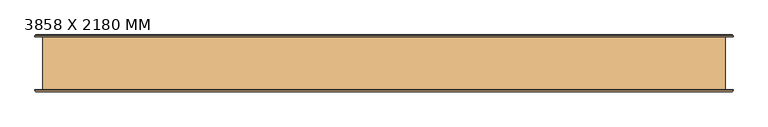
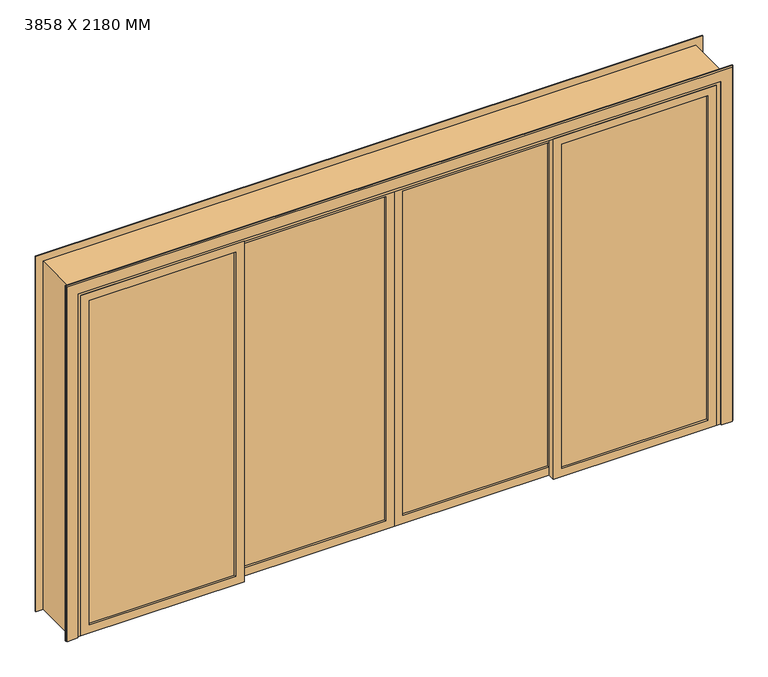
"""IFC4 building model written with IfcOpenShell, lengths in millimetres: door geometry, Porta envidraçada de correr quádrupla com revestimento : 3858 X 2180 MM."""

from ifc_helpers import new_model, si_unit, point, frame, frame_2d, origin, place, context, project, spatial, polyline, circle_curve, trimmed, segment, composite_curve, outline, extrude, faceted_brep, source, transform, mapped, element, save


def door_3858_x_2180_mm_a952f04c(model_context):
    return source(origin(), model_context, "Body", "SolidModel", [
        extrude(outline(composite_curve([segment(trimmed(circle_curve(frame_2d((990.0, 15.0)), 10.0), [point((1000.0, 15.0))], [point((990.0, 5.0))], False, "CARTESIAN"), True, "CONTINUOUS"), segment(polyline([(990.0, 5.0), (810.0, 5.0)]), True, "CONTINUOUS"), segment(trimmed(circle_curve(frame_2d((810.0, 15.0)), 10.0), [point((810.0, 5.0))], [point((800.0, 15.0))], False, "CARTESIAN"), True, "CONTINUOUS"), segment(polyline([(800.0, 15.0), (800.0, 35.0)]), True, "CONTINUOUS"), segment(trimmed(circle_curve(frame_2d((810.0, 35.0)), 10.0), [point((800.0, 35.0))], [point((810.0, 45.0))], False, "CARTESIAN"), True, "CONTINUOUS"), segment(polyline([(810.0, 45.0), (990.0, 45.0)]), True, "CONTINUOUS"), segment(trimmed(circle_curve(frame_2d((990.0, 35.0)), 10.0), [point((990.0, 45.0))], [point((1000.0, 35.0))], False, "CARTESIAN"), True, "CONTINUOUS"), segment(polyline([(1000.0, 35.0), (1000.0, 15.0)]), True, "CONTINUOUS")], self_intersect=False), holes=[composite_curve([segment(trimmed(circle_curve(frame_2d((985.0, 25.0)), 5.0), [point((985.0, 20.0))], [point((985.0, 30.0))], True, "CARTESIAN"), True, "CONTINUOUS"), segment(trimmed(circle_curve(frame_2d((985.0, 25.0)), 5.0), [point((985.0, 30.0))], [point((985.0, 20.0))], True, "CARTESIAN"), True, "CONTINUOUS")], self_intersect=False), composite_curve([segment(trimmed(circle_curve(frame_2d((815.0, 25.0)), 5.0), [point((815.0, 20.0))], [point((815.0, 30.0))], True, "CARTESIAN"), True, "CONTINUOUS"), segment(trimmed(circle_curve(frame_2d((815.0, 25.0)), 5.0), [point((815.0, 30.0))], [point((815.0, 20.0))], True, "CARTESIAN"), True, "CONTINUOUS")], self_intersect=False), composite_curve([segment(polyline([(960.0, 15.0), (960.0, 35.0)]), True, "CONTINUOUS"), segment(trimmed(circle_curve(frame_2d((955.0, 35.0)), 5.0), [point((960.0, 35.0))], [point((955.0, 40.0))], True, "CARTESIAN"), True, "CONTINUOUS"), segment(polyline([(955.0, 40.0), (845.0, 40.0)]), True, "CONTINUOUS"), segment(trimmed(circle_curve(frame_2d((845.0, 35.0)), 5.0), [point((845.0, 40.0))], [point((840.0, 35.0))], True, "CARTESIAN"), True, "CONTINUOUS"), segment(polyline([(840.0, 35.0), (840.0, 15.0)]), True, "CONTINUOUS"), segment(trimmed(circle_curve(frame_2d((845.0, 15.0)), 5.0), [point((840.0, 15.0))], [point((845.0, 10.0))], True, "CARTESIAN"), True, "CONTINUOUS"), segment(polyline([(845.0, 10.0), (955.0, 10.0)]), True, "CONTINUOUS"), segment(trimmed(circle_curve(frame_2d((955.0, 15.0)), 5.0), [point((955.0, 10.0))], [point((960.0, 15.0))], True, "CARTESIAN"), True, "CONTINUOUS")], self_intersect=False)]), frame((0.0, -65.0, 0.0), z_axis=(0.0, 1.0, 0.0), x_axis=(0.0, 0.0, 1.0)), (0.0, 0.0, 1.0), 3.0),
        extrude(outline(composite_curve([segment(trimmed(circle_curve(frame_2d((990.0, -35.0)), 10.0), [point((1000.0, -35.0))], [point((990.0, -45.0))], False, "CARTESIAN"), True, "CONTINUOUS"), segment(polyline([(990.0, -45.0), (810.0, -45.0)]), True, "CONTINUOUS"), segment(trimmed(circle_curve(frame_2d((810.0, -35.0)), 10.0), [point((810.0, -45.0))], [point((800.0, -35.0))], False, "CARTESIAN"), True, "CONTINUOUS"), segment(polyline([(800.0, -35.0), (800.0, -15.0)]), True, "CONTINUOUS"), segment(trimmed(circle_curve(frame_2d((810.0, -15.0)), 10.0), [point((800.0, -15.0))], [point((810.0, -5.0))], False, "CARTESIAN"), True, "CONTINUOUS"), segment(polyline([(810.0, -5.0), (990.0, -5.0)]), True, "CONTINUOUS"), segment(trimmed(circle_curve(frame_2d((990.0, -15.0)), 10.0), [point((990.0, -5.0))], [point((1000.0, -15.0))], False, "CARTESIAN"), True, "CONTINUOUS"), segment(polyline([(1000.0, -15.0), (1000.0, -35.0)]), True, "CONTINUOUS")], self_intersect=False), holes=[composite_curve([segment(trimmed(circle_curve(frame_2d((985.0, -25.0)), 5.0), [point((985.0, -30.0))], [point((985.0, -20.0))], True, "CARTESIAN"), True, "CONTINUOUS"), segment(trimmed(circle_curve(frame_2d((985.0, -25.0)), 5.0), [point((985.0, -20.0))], [point((985.0, -30.0))], True, "CARTESIAN"), True, "CONTINUOUS")], self_intersect=False), composite_curve([segment(trimmed(circle_curve(frame_2d((815.0, -25.0)), 5.0), [point((815.0, -30.0))], [point((815.0, -20.0))], True, "CARTESIAN"), True, "CONTINUOUS"), segment(trimmed(circle_curve(frame_2d((815.0, -25.0)), 5.0), [point((815.0, -20.0))], [point((815.0, -30.0))], True, "CARTESIAN"), True, "CONTINUOUS")], self_intersect=False), composite_curve([segment(polyline([(960.0, -35.0), (960.0, -15.0)]), True, "CONTINUOUS"), segment(trimmed(circle_curve(frame_2d((955.0, -15.0)), 5.0), [point((960.0, -15.0))], [point((955.0, -10.0))], True, "CARTESIAN"), True, "CONTINUOUS"), segment(polyline([(955.0, -10.0), (845.0, -10.0)]), True, "CONTINUOUS"), segment(trimmed(circle_curve(frame_2d((845.0, -15.0)), 5.0), [point((845.0, -10.0))], [point((840.0, -15.0))], True, "CARTESIAN"), True, "CONTINUOUS"), segment(polyline([(840.0, -15.0), (840.0, -35.0)]), True, "CONTINUOUS"), segment(trimmed(circle_curve(frame_2d((845.0, -35.0)), 5.0), [point((840.0, -35.0))], [point((845.0, -40.0))], True, "CARTESIAN"), True, "CONTINUOUS"), segment(polyline([(845.0, -40.0), (955.0, -40.0)]), True, "CONTINUOUS"), segment(trimmed(circle_curve(frame_2d((955.0, -35.0)), 5.0), [point((955.0, -40.0))], [point((960.0, -35.0))], True, "CARTESIAN"), True, "CONTINUOUS")], self_intersect=False)]), frame((0.0, -65.0, 0.0), z_axis=(0.0, 1.0, 0.0), x_axis=(0.0, 0.0, 1.0)), (0.0, 0.0, 1.0), 3.0),
        extrude(outline(polyline([(2130.0, -964.5), (0.0, -964.5), (0.0, 0.0), (2130.0, 0.0), (2130.0, -964.5)]), holes=[polyline([(2080.0, -50.0), (50.0, -50.0), (50.0, -914.5), (2080.0, -914.5), (2080.0, -50.0)])]), frame((0.0, -105.0, 0.0), z_axis=(0.0, 1.0, 0.0), x_axis=(0.0, 0.0, 1.0)), (0.0, 0.0, 1.0), 40.0),
        extrude(outline(polyline([(2130.0, 914.5), (0.0, 914.5), (0.0, 1879.0), (2130.0, 1879.0), (2130.0, 914.5)]), holes=[polyline([(2080.0, 1829.0), (50.0, 1829.0), (50.0, 964.5), (2080.0, 964.5), (2080.0, 1829.0)])]), frame((0.0, -150.0, 0.0), z_axis=(0.0, 1.0, 0.0), x_axis=(0.0, 0.0, 1.0)), (0.0, 0.0, 1.0), 40.0),
        extrude(outline(polyline([(2130.0, 0.0), (0.0, 0.0), (0.0, 964.5), (2130.0, 964.5), (2130.0, 0.0)]), holes=[polyline([(2080.0, 914.5), (50.0, 914.5), (50.0, 50.0), (2080.0, 50.0), (2080.0, 914.5)])]), frame((0.0, -105.0, 0.0), z_axis=(0.0, 1.0, 0.0), x_axis=(0.0, 0.0, 1.0)), (0.0, 0.0, 1.0), 40.0),
        extrude(outline(polyline([(2130.0, -1879.0), (0.0, -1879.0), (0.0, -914.5), (2130.0, -914.5), (2130.0, -1879.0)]), holes=[polyline([(2080.0, -964.5), (50.0, -964.5), (50.0, -1829.0), (2080.0, -1829.0), (2080.0, -964.5)])]), frame((0.0, -150.0, 0.0), z_axis=(0.0, 1.0, 0.0), x_axis=(0.0, 0.0, 1.0)), (0.0, 0.0, 1.0), 40.0),
        extrude(outline(polyline([(0.0, 1879.0), (0.0, 1929.0), (2180.0, 1929.0), (2180.0, -1929.0), (0.0, -1929.0), (0.0, -1879.0), (2130.0, -1879.0), (2130.0, 1879.0), (0.0, 1879.0)])), frame((0.0, -150.0, 0.0), z_axis=(0.0, 1.0, 0.0), x_axis=(0.0, 0.0, 1.0)), (0.0, 0.0, 1.0), 300.0),
        extrude(outline(polyline([(914.5, -78.0), (914.5, -92.0), (50.0, -92.0), (50.0, -78.0), (914.5, -78.0)])), frame((0.0, 0.0, 50.0), z_axis=(0.0, 0.0, 1.0), x_axis=(1.0, 0.0, 0.0)), (0.0, 0.0, 1.0), 2030.0),
        extrude(outline(polyline([(1829.0, -123.0), (1829.0, -137.0), (964.5, -137.0), (964.5, -123.0), (1829.0, -123.0)])), frame((0.0, 0.0, 50.0), z_axis=(0.0, 0.0, 1.0), x_axis=(1.0, 0.0, 0.0)), (0.0, 0.0, 1.0), 2030.0),
        extrude(outline(polyline([(-964.5, -123.0), (-964.5, -137.0), (-1829.0, -137.0), (-1829.0, -123.0), (-964.5, -123.0)])), frame((0.0, 0.0, 50.0), z_axis=(0.0, 0.0, 1.0), x_axis=(1.0, 0.0, 0.0)), (0.0, 0.0, 1.0), 2030.0),
        extrude(outline(polyline([(-50.0, -78.0), (-50.0, -92.0), (-914.5, -92.0), (-914.5, -78.0), (-50.0, -78.0)])), frame((0.0, 0.0, 50.0), z_axis=(0.0, 0.0, 1.0), x_axis=(1.0, 0.0, 0.0)), (0.0, 0.0, 1.0), 2030.0),
        extrude(outline(polyline([(-964.5, -123.0), (-964.5, -137.0), (-1829.0, -137.0), (-1829.0, -123.0), (-964.5, -123.0)])), frame((0.0, 0.0, 50.0), z_axis=(0.0, 0.0, 1.0), x_axis=(1.0, 0.0, 0.0)), (0.0, 0.0, 1.0), 2030.0),
        extrude(outline(polyline([(-50.0, -78.0), (-50.0, -92.0), (-914.5, -92.0), (-914.5, -78.0), (-50.0, -78.0)])), frame((0.0, 0.0, 50.0), z_axis=(0.0, 0.0, 1.0), x_axis=(1.0, 0.0, 0.0)), (0.0, 0.0, 1.0), 2030.0),
        extrude(outline(polyline([(964.5, -123.0), (1829.0, -123.0), (1829.0, -137.0), (964.5, -137.0), (964.5, -123.0)])), frame((0.0, 0.0, 50.0), z_axis=(0.0, 0.0, 1.0), x_axis=(1.0, 0.0, 0.0)), (0.0, 0.0, 1.0), 2030.0),
        extrude(outline(polyline([(50.0, -78.0), (914.5, -78.0), (914.5, -92.0), (50.0, -92.0), (50.0, -78.0)])), frame((0.0, 0.0, 50.0), z_axis=(0.0, 0.0, 1.0), x_axis=(1.0, 0.0, 0.0)), (0.0, 0.0, 1.0), 2030.0),
        faceted_brep([(1972.0, 154.0, 0.0), (1972.0, 150.0, 0.0), (1902.0, 150.0, 0.0), (1902.0, 160.0, 0.0), (1966.0, 160.0, 0.0), (1972.0, 154.0, 2223.0), (1972.0, 150.0, 2223.0), (-1972.0, 150.0, 2223.0), (-1972.0, 150.0, 0.0), (-1902.0, 150.0, 0.0), (-1902.0, 150.0, 2153.0), (1902.0, 150.0, 2153.0), (1902.0, 160.0, 2153.0), (-1902.0, 160.0, 2153.0), (-1902.0, 160.0, 0.0), (-1966.0, 160.0, 0.0), (-1966.0, 160.0, 2217.0), (1966.0, 160.0, 2217.0), (-1972.0, 154.0, 0.0), (-1972.0, 154.0, 2223.0)], [[[0, 1, 2, 3, 4]], [[1, 0, 5, 6]], [[2, 1, 6, 7, 8, 9, 10, 11]], [[3, 2, 11, 12]], [[4, 3, 12, 13, 14, 15, 16, 17]], [[0, 4, 17, 5]], [[13, 10, 9, 14]], [[18, 15, 14, 9, 8]], [[19, 16, 15, 18]], [[7, 19, 18, 8]], [[5, 17, 16, 19]], [[12, 11, 10, 13]], [[6, 5, 19, 7]]]),
        faceted_brep([(1972.0, -154.0, 0.0), (1966.0, -160.0, 0.0), (1902.0, -160.0, 0.0), (1902.0, -150.0, 0.0), (1972.0, -150.0, 0.0), (1972.0, -154.0, 2223.0), (1966.0, -160.0, 2217.0), (-1966.0, -160.0, 2217.0), (-1966.0, -160.0, 0.0), (-1902.0, -160.0, 0.0), (-1902.0, -160.0, 2153.0), (1902.0, -160.0, 2153.0), (1902.0, -150.0, 2153.0), (-1902.0, -150.0, 2153.0), (-1902.0, -150.0, 0.0), (-1972.0, -150.0, 0.0), (-1972.0, -150.0, 2223.0), (1972.0, -150.0, 2223.0), (-1972.0, -154.0, 2223.0), (-1972.0, -154.0, 0.0)], [[[0, 1, 2, 3, 4]], [[1, 0, 5, 6]], [[2, 1, 6, 7, 8, 9, 10, 11]], [[3, 2, 11, 12]], [[4, 3, 12, 13, 14, 15, 16, 17]], [[0, 4, 17, 5]], [[7, 18, 19, 8]], [[19, 15, 14, 9, 8]], [[13, 10, 9, 14]], [[18, 16, 15, 19]], [[6, 5, 18, 7]], [[12, 11, 10, 13]], [[5, 17, 16, 18]]]),
    ])


if __name__ == "__main__":
    model = new_model("IFC4")
    model_context = context("Model", 3, world=origin())
    ifc_project = project(units=[si_unit("LENGTHUNIT", "METRE", prefix="MILLI")], contexts=[model_context])
    site = spatial("IfcSite", under=ifc_project)
    building = spatial("IfcBuilding", under=site)
    placement = place(None, origin())
    door_3858_x_2180_mm_shape = door_3858_x_2180_mm_a952f04c(model_context)
    element("IfcDoor", 1, ObjectType="Porta envidraçada de correr quádrupla com revestimento : 3858 X 2180 MM", at=placement, inside=building, context=model_context, shape_type="MappedRepresentation", body=[
        mapped(door_3858_x_2180_mm_shape, transform((0.0, 0.0, 0.0), x_axis=(1.0, 0.0, 0.0), y_axis=(0.0, 1.0, 0.0), z_axis=(0.0, 0.0, 1.0))),
    ])
    save(model, "model.ifc")

# Revit data of these elements
# Type "Porta envidraçada de correr quádrupla com revestimento : 3858 X 2180 MM"
#   Type Mark = "49"
#   Construction Type Id = "GSP4R"
#   Analytic Construction = "Vidraça única Pilkington 1/8 pol"
#   Visual Light Transmittance = 0.9
#   Thermal Resistance (R) = 0.271106 (m²·K)/W
#   Largura da apara = 0.070 m
#   Espessura da apara = 0.010 m
#   Solar Heat Gain Coefficient = 0.78
#   Rough Width = 3.858 m
#   Rough Height = 2.180 m
#   Largura da moldura do painel = 0.050 m
#   Espessura da moldura do painel = 0.040 m
#   Heat Transfer Coefficient (U) = 3.6886 W/(m²·K)
#   Largura do puxador = 0.040 m
#   Altura do puxador = 0.200 m
#   Largura da estrutura = 0.050 m
#   Height = 2.180 m
#   Width = 3.858 m
#   Define Thermal Properties by = 1
#   Function = 1
#   Material da apara = none
#   Material do puxador = none
#   Vidro = none
#   Material da moldura = none
#   Thickness = 0
#   Wall Closure = (empty or 0)
# Element 1 (IfcDoor, "Porta envidraçada de correr quádrupla com revestimento : 3858 X 2180 MM")
#   Materials on its faces: "Vidro"
# Materials
#   "Vidro": class "Vidro", colour RGB 0 128 192, transparency 0.9, Description = "Vidro de sílica", Cost = 0
